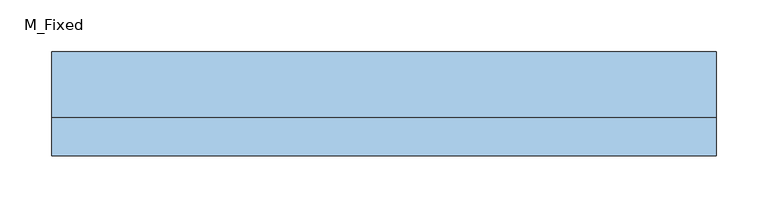
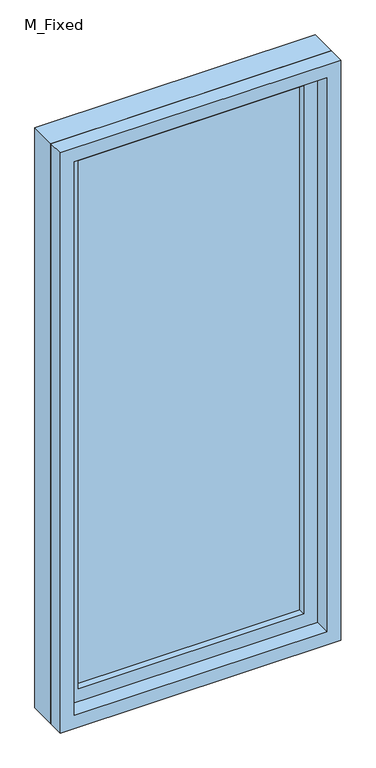
"""IFC4 building model written with IfcOpenShell, lengths in millimetres: window geometry, M_Fixed : 1400 x 640 Ahşap."""

from ifc_helpers import new_model, si_unit, frame, origin, place, context, project, spatial, polyline, outline, extrude, source, transform, mapped, element, save


def m_fixed_27182cef(model_context):
    return source(origin(), model_context, "Body", "SweptSolid", [
        extrude(outline(polyline([(-257.0, 28.0), (257.0, 28.0), (257.0, 16.0), (-257.0, 16.0), (-257.0, 28.0)])), frame((0.0, 0.0, 978.0), z_axis=(0.0, 0.0, 1.0), x_axis=(1.0, 0.0, 0.0)), (0.0, 0.0, 1.0), 1274.0),
        extrude(outline(polyline([(2296.0, -301.0), (934.0, -301.0), (934.0, 301.0), (2296.0, 301.0), (2296.0, -301.0)]), holes=[polyline([(2252.0, -257.0), (2252.0, 257.0), (978.0, 257.0), (978.0, -257.0), (2252.0, -257.0)])]), frame((0.0, 0.0, 0.0), z_axis=(0.0, 1.0, 0.0), x_axis=(0.0, 0.0, 1.0)), (0.0, 0.0, 1.0), 44.0),
        extrude(outline(polyline([(2315.0, -320.0), (915.0, -320.0), (915.0, 320.0), (2315.0, 320.0), (2315.0, -320.0)]), holes=[polyline([(2296.0, -301.0), (2296.0, 301.0), (934.0, 301.0), (934.0, -301.0), (2296.0, -301.0)])]), frame((0.0, 0.0, 0.0), z_axis=(0.0, 1.0, 0.0), x_axis=(0.0, 0.0, 1.0)), (0.0, 0.0, 1.0), 63.0),
        extrude(outline(polyline([(2315.0, -320.0), (915.0, -320.0), (915.0, 320.0), (2315.0, 320.0), (2315.0, -320.0)]), holes=[polyline([(2283.0, -288.0), (2283.0, 288.0), (947.0, 288.0), (947.0, -288.0), (2283.0, -288.0)])]), frame((0.0, -37.0, 0.0), z_axis=(0.0, 1.0, 0.0), x_axis=(0.0, 0.0, 1.0)), (0.0, 0.0, 1.0), 37.0),
    ])


if __name__ == "__main__":
    model = new_model("IFC4")
    model_context = context("Model", 3, world=origin())
    ifc_project = project(units=[si_unit("LENGTHUNIT", "METRE", prefix="MILLI")], contexts=[model_context])
    site = spatial("IfcSite", under=ifc_project)
    building = spatial("IfcBuilding", under=site)
    placement = place(None, origin())
    m_fixed_shape = m_fixed_27182cef(model_context)
    element("IfcWindow", 1, ObjectType="M_Fixed : 1400 x 640 Ahşap", at=placement, inside=building, context=model_context, shape_type="MappedRepresentation", body=[
        mapped(m_fixed_shape, transform((0.0, 0.0, 0.0), x_axis=(1.0, 0.0, 0.0), y_axis=(0.0, 1.0, 0.0), z_axis=(0.0, 0.0, 1.0))),
    ])
    save(model, "model.ifc")

# Revit data of these elements
# Type "M_Fixed : 1400 x 640 Ahşap"
#   Type Mark = "27"
#   Construction Type Id = "GSP4R"
#   Analytic Construction = "1/8 in Pilkington single glazing"
#   Visual Light Transmittance = 0.9
#   Thermal Resistance (R) = 0.271106 (m²·K)/W
#   Solar Heat Gain Coefficient = 0.78
#   Heat Transfer Coefficient (U) = 3.6886 W/(m²·K)
#   Height = 140 cm
#   Default Sill Height = 91.5 cm
#   Width = 64 cm
#   Window Inset = 1.9 cm
#   Define Thermal Properties by = 1
#   Frame Exterior Material = Sash
#   Frame Interior Material = Sash
#   Glass Pane Material = Glass
#   Sash = Sash
#   Wall Closure = (empty or 0)
# Element 1 (IfcWindow, "M_Fixed : 1400 x 640 Ahşap")
#   Materials on its faces: "Sash", "Glass"
# Materials
#   "Sash": class "Wood", colour RGB 224 178 126, transparency 0, Cost = 0
#   "Glass": class "Glass", colour RGB 0 128 192, transparency 0.9, Description = "Soda Lime Glass", Cost = 0
